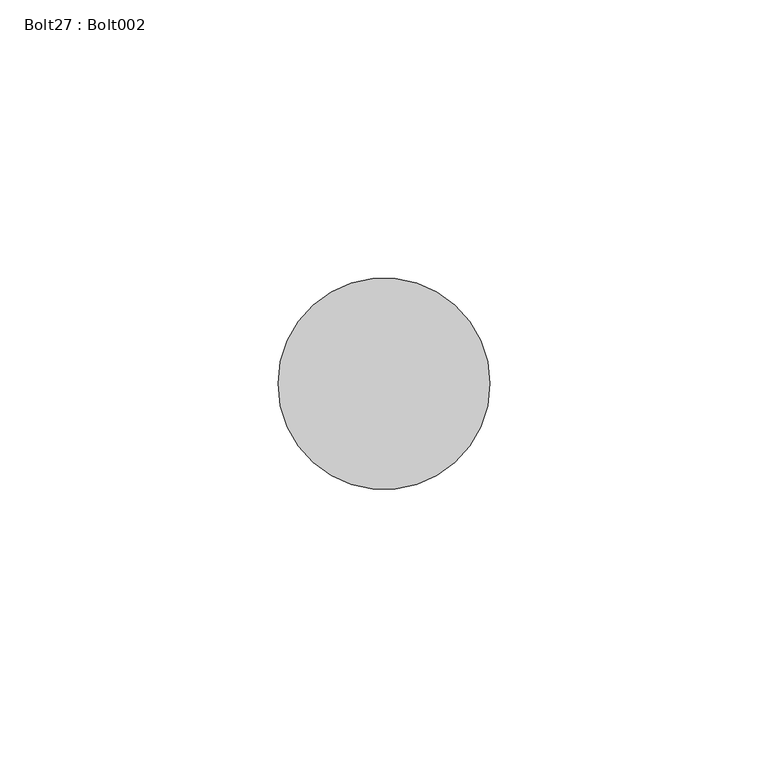
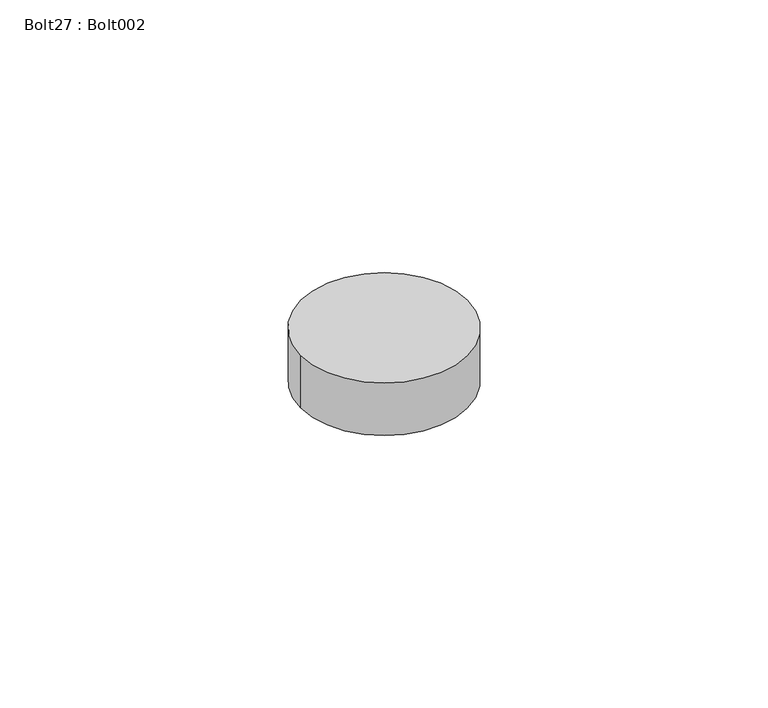
"""IFC4 building model written with IfcOpenShell, lengths in millimetres: proxy geometry, Bolt27 : Bolt002."""

from ifc_helpers import new_model, si_unit, point, frame, frame_2d, origin, place, context, project, spatial, circle_curve, trimmed, segment, composite_curve, outline, extrude, source, transform, mapped, element, save


def bolt27_bolt002_acca65bd(model_context):
    return source(origin(), model_context, "Body", "SweptSolid", [
        extrude(outline(composite_curve([segment(trimmed(circle_curve(frame_2d((5062.3346014, 1896.5882072)), 19.05), [point((5081.3846014, 1896.5882072))], [point((5043.2846014, 1896.5882072))], False, "CARTESIAN"), True, "CONTINUOUS"), segment(trimmed(circle_curve(frame_2d((5062.3346014, 1896.5882072)), 19.05), [point((5043.2846014, 1896.5882072))], [point((5081.3846014, 1896.5882072))], False, "CARTESIAN"), True, "CONTINUOUS")], self_intersect=False)), frame((0.0, 0.0, 36709.0959962), z_axis=(0.0, 0.0, 1.0), x_axis=(1.0, 0.0, 0.0)), (0.0, 0.0, 1.0), 12.7),
    ])


if __name__ == "__main__":
    model = new_model("IFC4")
    model_context = context("Model", 3, world=origin())
    ifc_project = project(units=[si_unit("LENGTHUNIT", "METRE", prefix="MILLI")], contexts=[model_context])
    site = spatial("IfcSite", under=ifc_project)
    building = spatial("IfcBuilding", under=site)
    placement = place(None, origin())
    bolt27_bolt002_shape = bolt27_bolt002_acca65bd(model_context)
    element("IfcBuildingElementProxy", 1, Name="Bolt27 : Bolt002", ObjectType="Bolt27 : Bolt002", at=placement, inside=building, context=model_context, shape_type="MappedRepresentation", body=[
        mapped(bolt27_bolt002_shape, transform((0.0, 0.0, 0.0), x_axis=(1.0, 0.0, 0.0), y_axis=(0.0, 1.0, 0.0), z_axis=(0.0, 0.0, 1.0))),
    ])
    save(model, "model.ifc")

# Revit data of these elements
# Type "Bolt27 : Bolt002"
#   NameOverride = "Bolt002"
# Element 1 (IfcBuildingElementProxy, "Bolt27 : Bolt002")
#   Materials on its faces: "STEEL ANGLE AND ANCHOR BOLT (SEE STRUCT. DWGS)"
# Materials
#   "STEEL ANGLE AND ANCHOR BOLT (SEE STRUCT. DWGS)": class "Unassigned", colour RGB 128 128 128, transparency 0, Cost = 0
